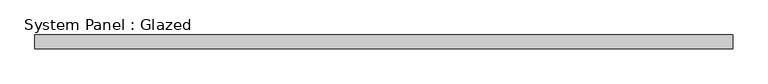
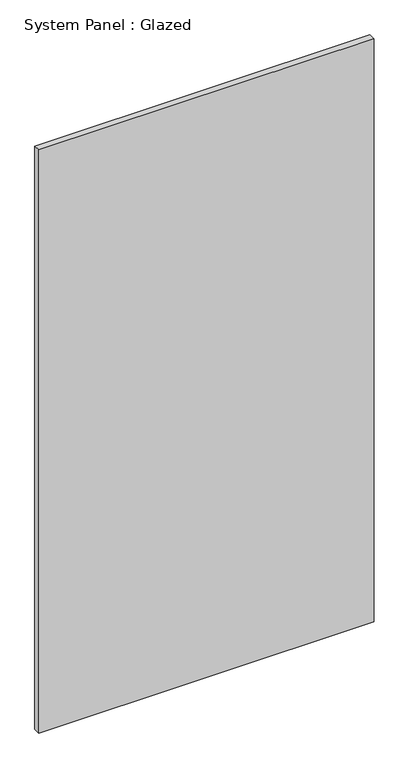
"""IFC4 building model written with IfcOpenShell, lengths in millimetres: plate geometry, System Panel : Glazed."""

from ifc_helpers import new_model, si_unit, origin, origin_with_axes, place, context, project, spatial, polyline, outline, extrude, source, transform, mapped, element, save


def system_panel_glazed_e4649fa4(model_context):
    return source(origin(), model_context, "Body", "SweptSolid", [
        extrude(outline(polyline([(632.4999999, 24.5), (-632.4999999, 24.5), (-632.4999999, 49.5), (632.4999999, 49.5), (632.4999999, 24.5)])), origin_with_axes(), (0.0, 0.0, 1.0), 2325.0),
    ])


if __name__ == "__main__":
    model = new_model("IFC4")
    model_context = context("Model", 3, world=origin())
    ifc_project = project(units=[si_unit("LENGTHUNIT", "METRE", prefix="MILLI")], contexts=[model_context])
    site = spatial("IfcSite", under=ifc_project)
    building = spatial("IfcBuilding", under=site)
    placement = place(None, origin())
    system_panel_glazed_shape = system_panel_glazed_e4649fa4(model_context)
    element("IfcPlate", 1, ObjectType="System Panel : Glazed", at=placement, inside=building, context=model_context, shape_type="MappedRepresentation", body=[
        mapped(system_panel_glazed_shape, transform((0.0, 0.0, 0.0), x_axis=(1.0, 0.0, 0.0), y_axis=(0.0, 1.0, 0.0), z_axis=(0.0, 0.0, 1.0))),
    ])
    save(model, "model.ifc")

# Revit data of these elements
# Type "System Panel : Glazed"
#   Construction Type Id = "GSP4R"
#   Analytic Construction = "1/8 in Pilkington single glazing"
#   Visual Light Transmittance = 0.9
#   Solar Heat Gain Coefficient = 0.86
#   Heat Transfer Coefficient (U) = 6.7069 W/(m²·K)
#   Define Thermal Properties by = 1
# Element 1 (IfcPlate, "System Panel : Glazed")
#   Materials on its faces: "Glass"
# Materials
#   "Glass": class "Glass", colour RGB 0 128 192, transparency 0.9, Description = "Soda Lime Glass", Cost = 0
